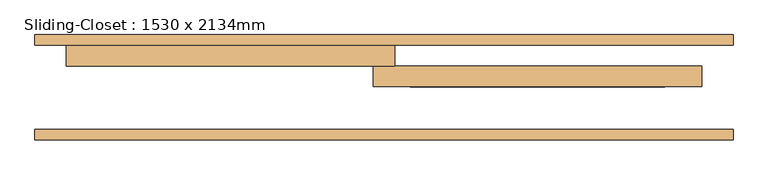
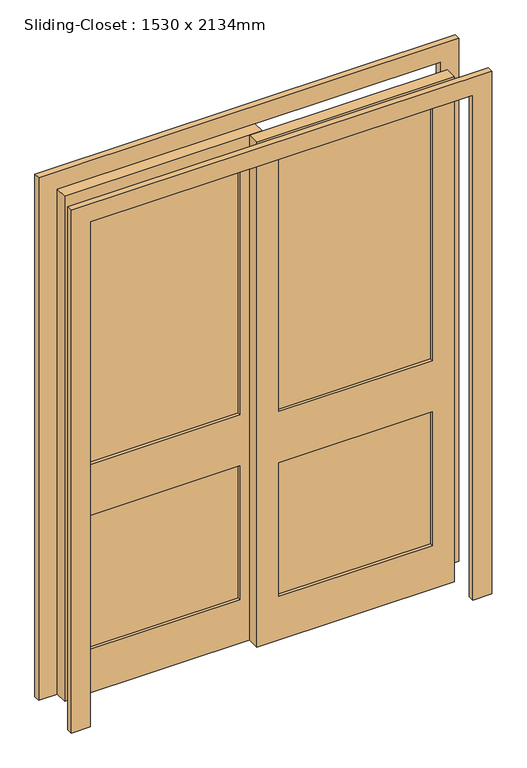
"""IFC4 building model written with IfcOpenShell, lengths in millimetres: door geometry, Sliding-Closet : 1530 x 2134mm."""

from ifc_helpers import new_model, si_unit, frame, origin, place, context, project, spatial, polyline, outline, extrude, source, transform, mapped, element, save


def sliding_closet_1530_x_2134mm_bff4d879(model_context):
    return source(origin(), model_context, "Body", "SweptSolid", [
        extrude(outline(polyline([(-63.5, 191.29375), (-676.0765625, 191.29375), (-676.0765625, 215.9), (-63.5, 215.9), (-63.5, 191.29375)])), frame((0.0, 0.0, 965.2), z_axis=(0.0, 0.0, 1.0), x_axis=(1.0, 0.0, 0.0)), (0.0, 0.0, 1.0), 1079.896875),
        extrude(outline(polyline([(-63.5, 191.29375), (-676.0765625, 191.29375), (-676.0765625, 215.9), (-63.5, 215.9), (-63.5, 191.29375)])), frame((0.0, 0.0, 184.15), z_axis=(0.0, 0.0, 1.0), x_axis=(1.0, 0.0, 0.0)), (0.0, 0.0, 1.0), 565.15),
        extrude(outline(polyline([(63.5, 165.89375), (676.0765625, 165.89375), (676.0765625, 141.2875), (63.5, 141.2875), (63.5, 165.89375)])), frame((0.0, 0.0, 965.2), z_axis=(0.0, 0.0, 1.0), x_axis=(1.0, 0.0, 0.0)), (0.0, 0.0, 1.0), 1079.896875),
        extrude(outline(polyline([(63.5, 165.89375), (676.0765625, 165.89375), (676.0765625, 141.2875), (63.5, 141.2875), (63.5, 165.89375)])), frame((0.0, 0.0, 184.15), z_axis=(0.0, 0.0, 1.0), x_axis=(1.0, 0.0, 0.0)), (0.0, 0.0, 1.0), 565.15),
        extrude(outline(polyline([(2133.996875, 25.4), (2133.996875, -764.9765625), (0.0, -764.9765625), (0.0, 25.4), (2133.996875, 25.4)]), holes=[polyline([(184.15, -676.0765625), (749.3, -676.0765625), (749.3, -63.5), (184.15, -63.5), (184.15, -676.0765625)]), polyline([(965.2, -676.0765625), (2045.096875, -676.0765625), (2045.096875, -63.5), (965.2, -63.5), (965.2, -676.0765625)])]), frame((0.0, 178.59375, 0.0), z_axis=(0.0, 1.0, 0.0), x_axis=(0.0, 0.0, 1.0)), (0.0, 0.0, 1.0), 50.00625),
        extrude(outline(polyline([(0.0, -839.9859375), (0.0, -764.9765625), (2133.996875, -764.9765625), (2133.996875, 764.9765625), (0.0, 764.9765625), (0.0, 839.9859375), (2209.00625, 839.9859375), (2209.00625, -839.9859375), (0.0, -839.9859375)])), frame((0.0, 0.396875, 0.0), z_axis=(0.0, 1.0, 0.0), x_axis=(0.0, 0.0, 1.0)), (0.0, 0.0, 1.0), 25.003125),
        extrude(outline(polyline([(0.0, 839.9859375), (2209.00625, 839.9859375), (2209.00625, -839.9859375), (0.0, -839.9859375), (0.0, -764.9765625), (2133.996875, -764.9765625), (2133.996875, 764.9765625), (0.0, 764.9765625), (0.0, 839.9859375)])), frame((0.0, 228.6, 0.0), z_axis=(0.0, 1.0, 0.0), x_axis=(0.0, 0.0, 1.0)), (0.0, 0.0, 1.0), 25.003125),
        extrude(outline(polyline([(2133.996875, -25.4), (0.0, -25.4), (0.0, 764.9765625), (2133.996875, 764.9765625), (2133.996875, -25.4)]), holes=[polyline([(965.2, 676.0765625), (965.2, 63.5), (2045.096875, 63.5), (2045.096875, 676.0765625), (965.2, 676.0765625)]), polyline([(184.15, 676.0765625), (184.15, 63.5), (749.3, 63.5), (749.3, 676.0765625), (184.15, 676.0765625)])]), frame((0.0, 128.5875, 0.0), z_axis=(0.0, 1.0, 0.0), x_axis=(0.0, 0.0, 1.0)), (0.0, 0.0, 1.0), 50.00625),
    ])


if __name__ == "__main__":
    model = new_model("IFC4")
    model_context = context("Model", 3, world=origin())
    ifc_project = project(units=[si_unit("LENGTHUNIT", "METRE", prefix="MILLI")], contexts=[model_context])
    site = spatial("IfcSite", under=ifc_project)
    building = spatial("IfcBuilding", under=site)
    placement = place(None, origin())
    sliding_closet_1530_x_2134mm_shape = sliding_closet_1530_x_2134mm_bff4d879(model_context)
    element("IfcDoor", 1, ObjectType="Sliding-Closet : 1530 x 2134mm", at=placement, inside=building, context=model_context, shape_type="MappedRepresentation", body=[
        mapped(sliding_closet_1530_x_2134mm_shape, transform((0.0, 0.0, 0.0), x_axis=(1.0, 0.0, 0.0), y_axis=(0.0, 1.0, 0.0), z_axis=(0.0, 0.0, 1.0))),
    ])
    save(model, "model.ifc")

# Revit data of these elements
# Type "Sliding-Closet : 1530 x 2134mm"
#   Type Mark = "56"
#   Assembly Code = "C1020"
#   Thickness = 0' - 1 31/32"
#   Height = 7' - 0 1/64"
#   Trim Projection Ext = 0' - 0 63/64"
#   Trim Projection Int = 0' - 0 63/64"
#   Trim Width = 0' - 2 61/64"
#   Width = 5' - 0 15/64"
#   Define Thermal Properties by = 0
#   Function = 0
#   Door Material = Door - Panel
#   Frame Material = Door - Frame
#   Wall Closure = (empty or 0)
# Element 1 (IfcDoor, "Sliding-Closet : 1530 x 2134mm")
#   Materials on its faces: "Door - Panel", "Door - Frame"
# Materials
#   "Door - Panel": class "Wood", colour RGB 227 170 128, transparency 0, Cost = 0
#   "Door - Frame": class "Miscellaneous", colour RGB 153 76 43, transparency 0, Cost = 0
